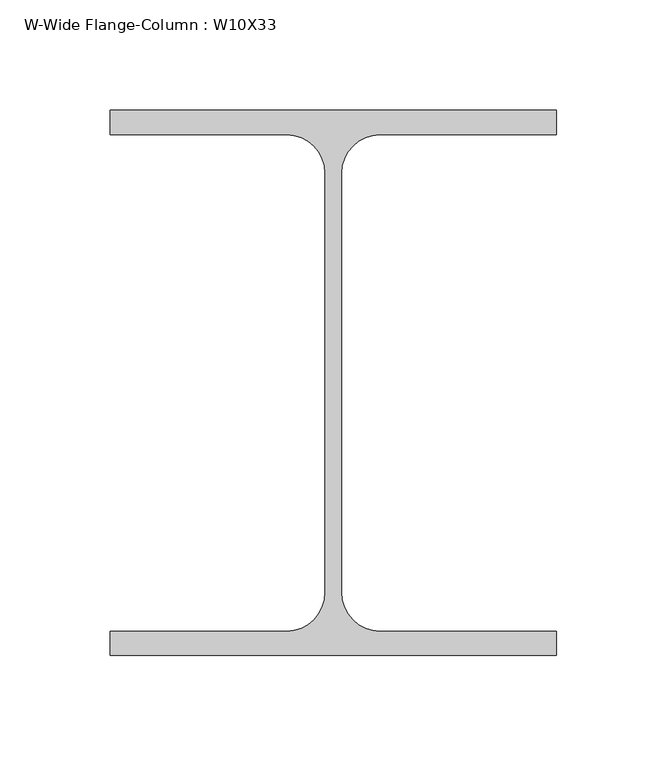
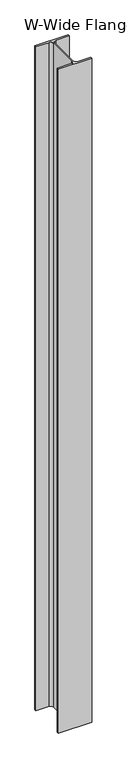
"""IFC4 building model written with IfcOpenShell, lengths in millimetres: column geometry, W-Wide Flange-Column : W10X33."""

from ifc_helpers import new_model, si_unit, point, frame, frame_2d, origin, place, context, project, spatial, polyline, circle_curve, trimmed, segment, composite_curve, outline, extrude, source, transform, mapped, element, save


def w_wide_flange_column_w10x33_823203b9(model_context):
    return source(origin(), model_context, "Body", "SweptSolid", [
        extrude(outline(composite_curve([segment(polyline([(101.092, 123.571), (101.092, 112.522), (21.209, 112.522)]), True, "CONTINUOUS"), segment(trimmed(circle_curve(frame_2d((21.209, 94.996)), 17.526), [point((21.209, 112.522))], [point((3.683, 94.996))], True, "CARTESIAN"), True, "CONTINUOUS"), segment(polyline([(3.683, 94.996), (3.683, -94.996)]), True, "CONTINUOUS"), segment(trimmed(circle_curve(frame_2d((21.209, -94.996)), 17.526), [point((3.683, -94.996))], [point((21.209, -112.522))], True, "CARTESIAN"), True, "CONTINUOUS"), segment(polyline([(21.209, -112.522), (101.092, -112.522), (101.092, -123.571), (-101.092, -123.571), (-101.092, -112.522), (-21.209, -112.522)]), True, "CONTINUOUS"), segment(trimmed(circle_curve(frame_2d((-21.209, -94.996)), 17.526), [point((-21.209, -112.522))], [point((-3.683, -94.996))], True, "CARTESIAN"), True, "CONTINUOUS"), segment(polyline([(-3.683, -94.996), (-3.683, 94.996)]), True, "CONTINUOUS"), segment(trimmed(circle_curve(frame_2d((-21.209, 94.996)), 17.526), [point((-3.683, 94.996))], [point((-21.209, 112.522))], True, "CARTESIAN"), True, "CONTINUOUS"), segment(polyline([(-21.209, 112.522), (-101.092, 112.522), (-101.092, 123.571), (101.092, 123.571)]), True, "CONTINUOUS")], self_intersect=False)), frame((0.0, 0.0, 23317.2), z_axis=(0.0, 0.0, 1.0), x_axis=(1.0, 0.0, 0.0)), (0.0, 0.0, 1.0), 4267.2),
    ])


if __name__ == "__main__":
    model = new_model("IFC4")
    model_context = context("Model", 3, world=origin())
    ifc_project = project(units=[si_unit("LENGTHUNIT", "METRE", prefix="MILLI")], contexts=[model_context])
    site = spatial("IfcSite", under=ifc_project)
    building = spatial("IfcBuilding", under=site)
    placement = place(None, origin())
    w_wide_flange_column_w10x33_shape = w_wide_flange_column_w10x33_823203b9(model_context)
    element("IfcColumn", 1, ObjectType="W-Wide Flange-Column : W10X33", at=placement, inside=building, context=model_context, shape_type="MappedRepresentation", body=[
        mapped(w_wide_flange_column_w10x33_shape, transform((0.0, 0.0, 0.0), x_axis=(1.0, 0.0, 0.0), y_axis=(0.0, 1.0, 0.0), z_axis=(0.0, 0.0, 1.0))),
    ])
    save(model, "model.ifc")

# Revit data of these elements
# Type "W-Wide Flange-Column : W10X33"
#   Assembly Code = "B10"
#   W = 33
#   bf = 0' - 7.96"
#   d = 0' - 9.73"
#   k = 0' - 1 1/8"
#   kr = 0' - 0.69"
#   tf = 0' - 0.435"
#   tw = 0' - 0.29"
#   A = 0.0674306 SF
#   Structural Material [instance default] = Steel ASTM A992
# Element 1 (IfcColumn, "W-Wide Flange-Column : W10X33")
#   Materials on its faces: "Steel ASTM A992"
# Materials
#   "Steel ASTM A992": class "Metal", colour RGB 199 199 199, transparency 0, Description = "Structural steel 50ksi", Cost = 0
